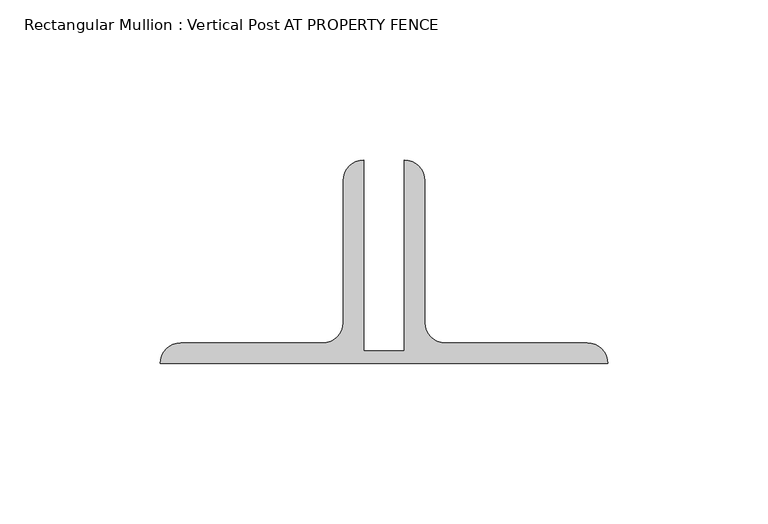
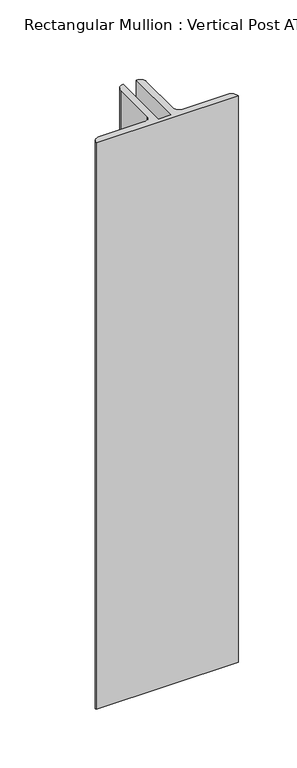
"""IFC4 building model written with IfcOpenShell, lengths in millimetres: member geometry, Rectangular Mullion : Vertical Post AT PROPERTY FENCE."""

from ifc_helpers import new_model, si_unit, point, frame, frame_2d, origin, place, context, project, spatial, polyline, circle_curve, trimmed, segment, composite_curve, outline, extrude, source, transform, mapped, element, save


def rectangular_mullion_vertical_post_at_property_fence_7ddc0c2c(model_context):
    return source(origin(), model_context, "Body", "SweptSolid", [
        extrude(outline(composite_curve([segment(polyline([(-6.35, 22.9145205), (6.35, 22.9145205), (6.35, 82.55)]), True, "CONTINUOUS"), segment(trimmed(circle_curve(frame_2d((6.35, 76.2)), 6.35), [point((6.35, 82.55))], [point((12.7, 76.2))], False, "CARTESIAN"), True, "CONTINUOUS"), segment(polyline([(12.7, 76.2), (12.7, 31.75)]), True, "CONTINUOUS"), segment(trimmed(circle_curve(frame_2d((19.05, 31.75)), 6.35), [point((12.7, 31.75))], [point((19.05, 25.4))], True, "CARTESIAN"), True, "CONTINUOUS"), segment(polyline([(19.05, 25.4), (63.5, 25.4)]), True, "CONTINUOUS"), segment(trimmed(circle_curve(frame_2d((63.5, 19.05)), 6.35), [point((63.5, 25.4))], [point((69.85, 19.05))], False, "CARTESIAN"), True, "CONTINUOUS"), segment(polyline([(69.85, 19.05), (-69.85, 19.05)]), True, "CONTINUOUS"), segment(trimmed(circle_curve(frame_2d((-63.5, 19.05)), 6.35), [point((-69.85, 19.05))], [point((-63.5, 25.4))], False, "CARTESIAN"), True, "CONTINUOUS"), segment(polyline([(-63.5, 25.4), (-19.05, 25.4)]), True, "CONTINUOUS"), segment(trimmed(circle_curve(frame_2d((-19.05, 31.75)), 6.35), [point((-19.05, 25.4))], [point((-12.7, 31.75))], True, "CARTESIAN"), True, "CONTINUOUS"), segment(polyline([(-12.7, 31.75), (-12.7, 76.2)]), True, "CONTINUOUS"), segment(trimmed(circle_curve(frame_2d((-6.35, 76.2)), 6.35), [point((-12.7, 76.2))], [point((-6.35, 82.55))], False, "CARTESIAN"), True, "CONTINUOUS"), segment(polyline([(-6.35, 82.55), (-6.35, 22.9145205)]), True, "CONTINUOUS")], self_intersect=False)), frame((0.0, 0.0, -588.8534967), z_axis=(0.0, 0.0, 1.0), x_axis=(1.0, 0.0, 0.0)), (0.0, 0.0, 1.0), 588.8534967),
    ])


if __name__ == "__main__":
    model = new_model("IFC4")
    model_context = context("Model", 3, world=origin())
    ifc_project = project(units=[si_unit("LENGTHUNIT", "METRE", prefix="MILLI")], contexts=[model_context])
    site = spatial("IfcSite", under=ifc_project)
    building = spatial("IfcBuilding", under=site)
    placement = place(None, origin())
    rectangular_mullion_vertical_post_at_property_fence_shape = rectangular_mullion_vertical_post_at_property_fence_7ddc0c2c(model_context)
    element("IfcMember", 1, ObjectType="Rectangular Mullion : Vertical Post AT PROPERTY FENCE", at=placement, inside=building, context=model_context, shape_type="MappedRepresentation", body=[
        mapped(rectangular_mullion_vertical_post_at_property_fence_shape, transform((0.0, 0.0, 0.0), x_axis=(1.0, 0.0, 0.0), y_axis=(0.0, 1.0, 0.0), z_axis=(0.0, 0.0, 1.0))),
    ])
    save(model, "model.ifc")

# Revit data of these elements
# Type "Rectangular Mullion : Vertical Post AT PROPERTY FENCE"
#   built-in parameter 1007351 = -0.0625 (stored number, unit not read)
#   built-in parameter 1007322 = 0.0126789 (stored number, unit not read)
#   built-in parameter 1007321 = 0.229167 (stored number, unit not read)
#   built-in parameter 1007320 = 0.229167 (stored number, unit not read)
# Element 1 (IfcMember, "Rectangular Mullion : Vertical Post AT PROPERTY FENCE")
#   Materials on its faces: "MAIN FENCE POST: (2) BACK/BACK GALVANIZED ANGLES (2) L2 1/2 X 2 1/2 X 1/4\") ANCHORED TO 8\"W X 42\" DEEP CONCRETE FOOTING(1)"
# Materials
#   "MAIN FENCE POST: (2) BACK/BACK GALVANIZED ANGLES (2) L2 1/2 X 2 1/2 X 1/4\") ANCHORED TO 8\"W X 42\" DEEP CONCRETE FOOTING(1)": class "Unassigned", colour RGB 211 211 211, transparency 0, Cost = 0
